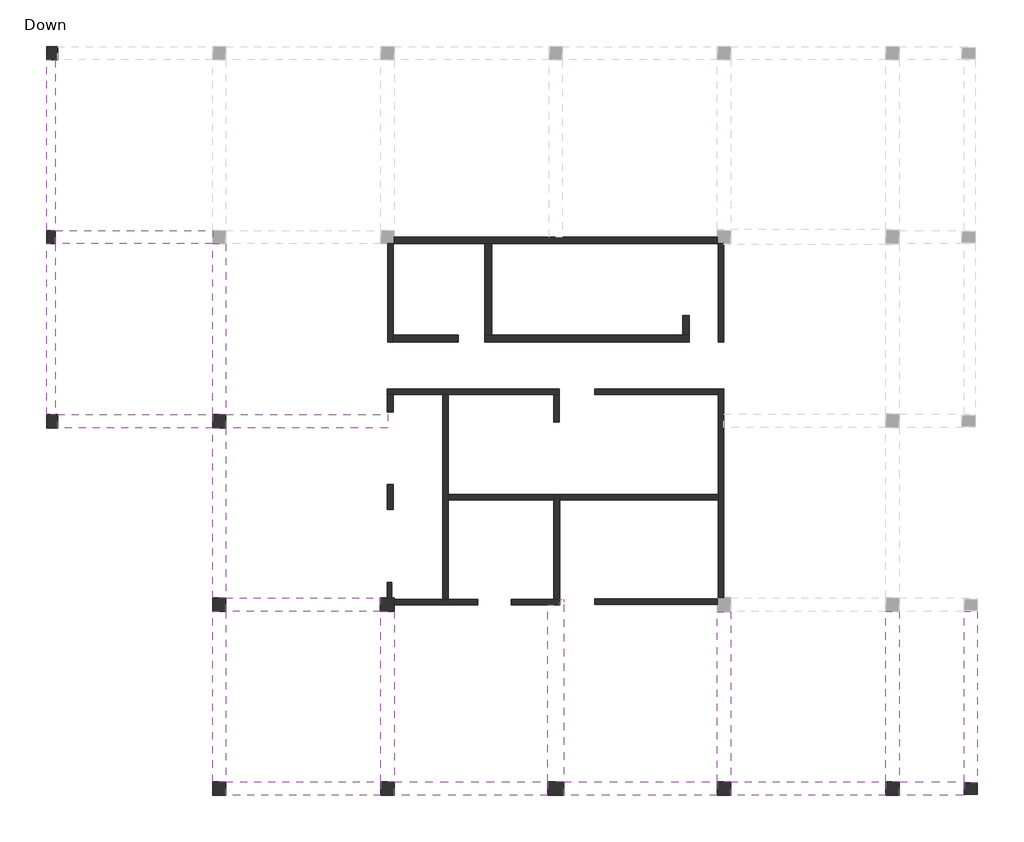
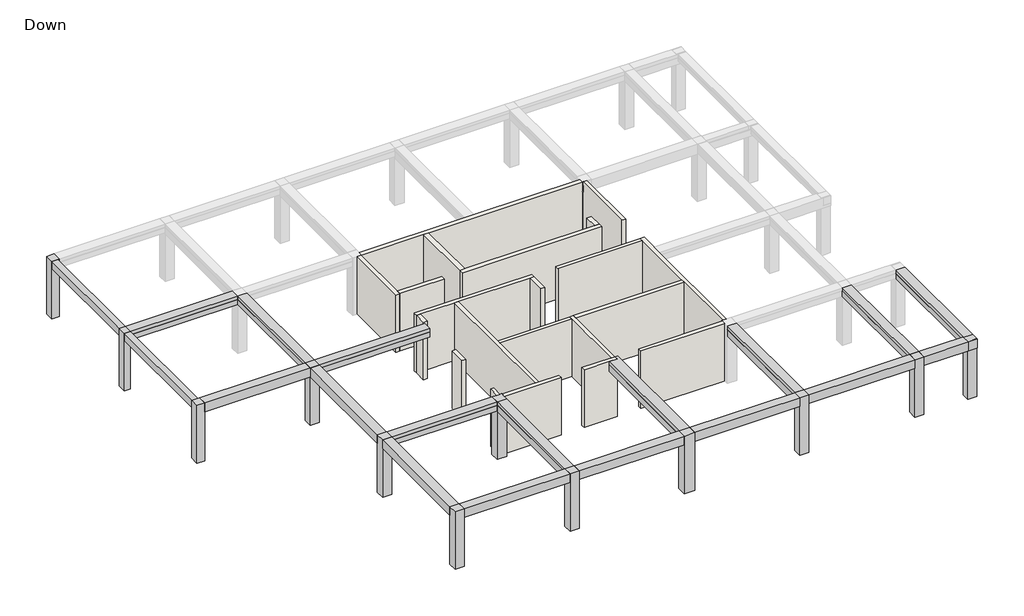
# One storey, part 1 of 2: 21 walls, 19 beams, 12 columns.
"""IFC4 building model written with IfcOpenShell, lengths in millimetres."""

from ifc_helpers import new_model, si_unit, frame, origin, origin_with_axes, place, context, project, spatial, polyline, outline, extrude, faceted_brep, element, save

model = new_model("IFC4")

# Units and contexts
model_context = context("Model", 3, world=origin())
ifc_project = project(units=[si_unit("LENGTHUNIT", "METRE", prefix="MILLI")], contexts=[model_context])

# Site, building, storey
site = spatial("IfcSite", under=ifc_project)
building = spatial("IfcBuilding", under=site)
storey = spatial("IfcBuildingStorey", under=building, Name="Down", Elevation=0.0)

# Beams
placement = place(None, origin())
element("IfcBeam", 1, ObjectType="Concrete Rectengular Beam : 40/50", at=placement, inside=storey, context=model_context, shape_type="SweptSolid", body=[
    extrude(outline(polyline([(4000.0, -21394.7160223), (3500.0, -21394.7160223), (3500.0, -20994.7160223), (3770.0, -20994.7160223), (3770.0, -20999.7160223), (4000.0, -20999.7160223), (4000.0, -21394.7160223)])), frame((0.0, 17936.6191558, 0.0), z_axis=(0.0, 1.0, 0.0), x_axis=(0.0, 0.0, 1.0)), (0.0, 0.0, 1.0), 7656.3440805),
])
element("IfcBeam", 2, ObjectType="Concrete Rectengular Beam : 40/50", at=placement, inside=storey, context=model_context, shape_type="SweptSolid", body=[
    extrude(outline(polyline([(4000.0, -21394.7160223), (3500.0, -21394.7160223), (3500.0, -20994.7160223), (3770.0, -20994.7160223), (3770.0, -20999.7160223), (4000.0, -20999.7160223), (4000.0, -21394.7160223)])), frame((0.0, 9666.6131842, 0.0), z_axis=(0.0, 1.0, 0.0), x_axis=(0.0, 0.0, 1.0)), (0.0, 0.0, 1.0), 7670.0059716),
])
element("IfcBeam", 3, ObjectType="Concrete Rectengular Beam : 60/60", at=placement, inside=storey, context=model_context, shape_type="SweptSolid", body=[
    extrude(outline(polyline([(3400.0, 16261.8802114), (3400.0, 16861.8802114), (3770.0, 16861.8802114), (3770.0, 16856.8802114), (4000.0, 16856.8802114), (4000.0, 16266.8802114), (3770.0, 16266.8802114), (3770.0, 16261.8802114), (3400.0, 16261.8802114)])), frame((0.0, -6825.0062825, 0.0), z_axis=(0.0, 1.0, 0.0), x_axis=(0.0, 0.0, 1.0)), (0.0, 0.0, 1.0), 7657.5072677),
])
element("IfcBeam", 4, ObjectType="Concrete Rectengular Beam : 60/60", at=placement, inside=storey, context=model_context, shape_type="SweptSolid", body=[
    extrude(outline(polyline([(-6825.0062825, 3400.0), (-7425.0062825, 3400.0), (-7425.0062825, 4000.0), (-6830.0062825, 4000.0), (-6830.0062825, 3770.0), (-6825.0062825, 3770.0), (-6825.0062825, 3400.0)])), frame((9303.3595467, 0.0, 0.0), z_axis=(1.0, 0.0, 0.0), x_axis=(0.0, 1.0, 0.0)), (0.0, 0.0, 1.0), 6958.5206647),
])
element("IfcBeam", 5, ObjectType="Concrete Rectengular Beam : 60/60", at=placement, inside=storey, context=model_context, shape_type="SweptSolid", body=[
    extrude(outline(polyline([(-6825.0062825, 3400.0), (-7425.0062825, 3400.0), (-7425.0062825, 4000.0), (-6830.0062825, 4000.0), (-6830.0062825, 3770.0), (-6825.0062825, 3770.0), (-6825.0062825, 3400.0)])), frame((1807.0810158, 0.0, 0.0), z_axis=(1.0, 0.0, 0.0), x_axis=(0.0, 1.0, 0.0)), (0.0, 0.0, 1.0), 6896.2785308),
])
element("IfcBeam", 6, ObjectType="Concrete Rectengular Beam : 60/60", at=placement, inside=storey, context=model_context, shape_type="SweptSolid", body=[
    extrude(outline(polyline([(-6825.0062825, 3400.0), (-7425.0062825, 3400.0), (-7425.0062825, 4000.0), (-6830.0062825, 4000.0), (-6830.0062825, 3770.0), (-6825.0062825, 3770.0), (-6825.0062825, 3400.0)])), frame((-5790.1585821, 0.0, 0.0), z_axis=(1.0, 0.0, 0.0), x_axis=(0.0, 1.0, 0.0)), (0.0, 0.0, 1.0), 6897.2395979),
])
element("IfcBeam", 7, ObjectType="Concrete Rectengular Beam : 60/60", at=placement, inside=storey, context=model_context, shape_type="SweptSolid", body=[
    extrude(outline(polyline([(-6825.0062825, 3400.0), (-7425.0062825, 3400.0), (-7425.0062825, 4000.0), (-6830.0062825, 4000.0), (-6830.0062825, 3770.0), (-6825.0062825, 3770.0), (-6825.0062825, 3400.0)])), frame((-13343.8144749, 0.0, 0.0), z_axis=(1.0, 0.0, 0.0), x_axis=(0.0, 1.0, 0.0)), (0.0, 0.0, 1.0), 6953.6558928),
])
element("IfcBeam", 8, ObjectType="Concrete Rectengular Beam : 60/60", at=placement, inside=storey, context=model_context, shape_type="SweptSolid", body=[
    extrude(outline(polyline([(4000.0, -13943.8144749), (3400.0, -13943.8144749), (3400.0, -13343.8144749), (3770.0, -13343.8144749), (3770.0, -13348.8144749), (4000.0, -13348.8144749), (4000.0, -13943.8144749)])), frame((0.0, -6825.0062825, 0.0), z_axis=(0.0, 1.0, 0.0), x_axis=(0.0, 0.0, 1.0)), (0.0, 0.0, 1.0), 7657.5072677),
])
element("IfcBeam", 9, ObjectType="Concrete Rectengular Beam : 60/60", at=placement, inside=storey, context=model_context, shape_type="SweptSolid", body=[
    extrude(outline(polyline([(3400.0, -13943.8144749), (3400.0, -13343.8144749), (3770.0, -13343.8144749), (3770.0, -13348.8144749), (4000.0, -13348.8144749), (4000.0, -13943.8144749), (3400.0, -13943.8144749)])), frame((0.0, 1432.5009852, 0.0), z_axis=(0.0, 1.0, 0.0), x_axis=(0.0, 0.0, 1.0)), (0.0, 0.0, 1.0), 7634.112199),
])
element("IfcBeam", 10, ObjectType="Concrete Rectengular Beam : 60/60", at=placement, inside=storey, context=model_context, shape_type="SweptSolid", body=[
    extrude(outline(polyline([(3400.0, -13943.8144749), (3400.0, -13343.8144749), (3770.0, -13343.8144749), (3770.0, -13348.8144749), (4000.0, -13348.8144749), (4000.0, -13938.8144749), (3770.0, -13938.8144749), (3770.0, -13943.8144749), (3400.0, -13943.8144749)])), frame((0.0, 9666.6131842, 0.0), z_axis=(0.0, 1.0, 0.0), x_axis=(0.0, 0.0, 1.0)), (0.0, 0.0, 1.0), 7670.0059716),
])
element("IfcBeam", 11, ObjectType="Concrete Rectengular Beam : 60/60", at=placement, inside=storey, context=model_context, shape_type="SweptSolid", body=[
    extrude(outline(polyline([(9666.6131842, 3400.0), (9066.6131842, 3400.0), (9066.6131842, 4000.0), (9661.6131842, 4000.0), (9661.6131842, 3770.0), (9666.6131842, 3770.0), (9666.6131842, 3400.0)])), frame((-20894.7160223, 0.0, 0.0), z_axis=(1.0, 0.0, 0.0), x_axis=(0.0, 1.0, 0.0)), (0.0, 0.0, 1.0), 6950.9015474),
])
element("IfcBeam", 12, ObjectType="Concrete Rectengular Beam : 60/60", at=placement, inside=storey, context=model_context, shape_type="SweptSolid", body=[
    extrude(outline(polyline([(17936.6191558, 3400.0), (17336.6191558, 3400.0), (17336.6191558, 3770.0), (17341.6191558, 3770.0), (17341.6191558, 4000.0), (17931.6191558, 4000.0), (17931.6191558, 3770.0), (17936.6191558, 3770.0), (17936.6191558, 3400.0)])), frame((-20994.7160223, 0.0, 0.0), z_axis=(1.0, 0.0, 0.0), x_axis=(0.0, 1.0, 0.0)), (0.0, 0.0, 1.0), 7050.9015474),
])
element("IfcBeam", 13, ObjectType="Concrete Rectengular Beam : 60/60", at=placement, inside=storey, context=model_context, shape_type="SweptSolid", body=[
    extrude(outline(polyline([(9666.6131842, 3400.0), (9066.6131842, 3400.0), (9066.6131842, 3770.0), (9071.6131842, 3770.0), (9071.6131842, 4000.0), (9661.6131842, 4000.0), (9661.6131842, 3770.0), (9666.6131842, 3770.0), (9666.6131842, 3400.0)])), frame((-13343.8144749, 0.0, 0.0), z_axis=(1.0, 0.0, 0.0), x_axis=(0.0, 1.0, 0.0)), (0.0, 0.0, 1.0), 7253.6558928),
])
element("IfcBeam", 14, ObjectType="Concrete Rectengular Beam : 60/60", at=placement, inside=storey, context=model_context, shape_type="SweptSolid", body=[
    extrude(outline(polyline([(1432.5009852, 3400.0), (832.5009852, 3400.0), (832.5009852, 3770.0), (837.5009852, 3770.0), (837.5009852, 4000.0), (1430.5203801, 4000.0), (1430.5203801, 3770.0), (1432.5009852, 3770.0), (1432.5009852, 3400.0)])), frame((-13343.8144749, 0.0, 0.0), z_axis=(1.0, 0.0, 0.0), x_axis=(0.0, 1.0, 0.0)), (0.0, 0.0, 1.0), 6919.0299628),
])
element("IfcBeam", 15, ObjectType="Concrete Rectengular Beam : 60/60", at=placement, inside=storey, context=model_context, shape_type="Brep", body=[
    faceted_brep([(19778.1411959, -7425.0062825, 4000.0), (20378.1412457, -7425.0062825, 4000.0), (20378.1616289, -7375.0062825, 4000.0), (19778.1615791, -7375.0062825, 4000.0), (19778.1411959, -7425.0062825, 3400.0), (19778.1615791, -7375.0062825, 3400.0), (20378.1412457, -7425.0062825, 3400.0), (20378.1616289, -7375.0062825, 3400.0)], [[[0, 1, 2, 3]], [[4, 0, 3, 5]], [[6, 4, 5, 7]], [[1, 6, 7, 2]], [[1, 0, 4, 6]], [[3, 2, 7, 5]]]),
    faceted_brep([(20381.5075349, 832.5009852, 3400.0), (19781.507485, 832.5009852, 3400.0), (19781.507485, 832.5009852, 3770.0), (19786.5074854, 832.5009852, 3770.0), (19786.5074854, 832.5009852, 4000.0), (20381.5075349, 832.5009852, 4000.0), (19778.3857943, -6825.0062825, 3770.0), (19778.383756, -6830.0062825, 3770.0), (19783.3837564, -6830.0062825, 3770.0), (19783.3837564, -6830.0062825, 4000.0), (19778.383756, -6830.0062825, 4000.0), (20378.365461, -6875.0062825, 4000.0), (19778.3654111, -6875.0062825, 4000.0), (19778.3654111, -6875.0062825, 3400.0), (20378.365461, -6875.0062825, 3400.0), (19778.3857943, -6825.0062825, 3400.0)], [[[0, 1, 2, 3, 4, 5]], [[2, 6, 7, 8, 3]], [[8, 9, 4, 3]], [[9, 8, 7, 10]], [[11, 12, 13, 14]], [[4, 9, 10, 12, 11, 5]], [[10, 7, 6, 2, 1, 15, 13, 12]], [[1, 0, 14, 13, 15]], [[0, 5, 11, 14]]]),
])
element("IfcBeam", 16, ObjectType="Concrete Rectengular Beam : 60/60", at=placement, inside=storey, context=model_context, shape_type="Brep", body=[
    faceted_brep([(16861.8802114, -7425.0062825, 4000.0), (19778.1411959, -7425.0062825, 4000.0), (19778.3654111, -6875.0062825, 4000.0), (19778.383756, -6830.0062825, 4000.0), (16861.8802114, -6830.0062825, 4000.0), (19778.3857943, -6825.0062825, 3400.0), (16861.8802114, -6825.0062825, 3400.0), (16861.8802114, -6825.0062825, 3770.0), (19778.3857943, -6825.0062825, 3770.0), (19778.3654111, -6875.0062825, 3400.0), (19778.1411959, -7425.0062825, 3400.0), (16861.8802114, -7425.0062825, 3400.0), (16861.8802114, -6830.0062825, 3770.0), (19778.383756, -6830.0062825, 3770.0)], [[[0, 1, 2, 3, 4]], [[5, 6, 7, 8]], [[5, 9, 10, 11, 6]], [[0, 11, 10, 1]], [[11, 0, 4, 12, 7, 6]], [[10, 9, 5, 8, 13, 3, 2, 1]], [[12, 13, 8, 7]], [[13, 12, 4, 3]]]),
])
element("IfcBeam", 17, ObjectType="Concrete Rectengular Beam : 60/70", at=placement, inside=storey, context=model_context, shape_type="SweptSolid", body=[
    extrude(outline(polyline([(3300.0, -6390.1585821), (3300.0, -5790.1585821), (3770.0, -5790.1585821), (3770.0, -5795.1585821), (4000.0, -5795.1585821), (4000.0, -6385.1585821), (3770.0, -6385.1585821), (3770.0, -6390.1585821), (3300.0, -6390.1585821)])), frame((0.0, -6825.0062825, 0.0), z_axis=(0.0, 1.0, 0.0), x_axis=(0.0, 0.0, 1.0)), (0.0, 0.0, 1.0), 7657.5072677),
])
element("IfcBeam", 18, ObjectType="Concrete Rectengular Beam : 60/70", at=placement, inside=storey, context=model_context, shape_type="SweptSolid", body=[
    extrude(outline(polyline([(3300.0, 8703.3595467), (3300.0, 9303.3595467), (3770.0, 9303.3595467), (3770.0, 9298.3595467), (4000.0, 9298.3595467), (4000.0, 8708.3595467), (3770.0, 8708.3595467), (3770.0, 8703.3595467), (3300.0, 8703.3595467)])), frame((0.0, -6825.0062825, 0.0), z_axis=(0.0, 1.0, 0.0), x_axis=(0.0, 0.0, 1.0)), (0.0, 0.0, 1.0), 7637.5072677),
])
element("IfcBeam", 19, ObjectType="Concrete Rectengular Beam : 70/70", at=placement, inside=storey, context=model_context, shape_type="Brep", body=[
    faceted_brep([(1807.0810158, 1138.5687304, 4000.0), (1807.0810158, 1377.9140303, 4000.0), (1628.3544453, 1377.9140303, 4000.0), (1628.3544453, 1127.9140303, 4000.0), (1112.0810158, 1127.9140303, 4000.0), (1112.0810158, -6825.0062825, 4000.0), (1802.0810158, -6825.0062825, 4000.0), (1802.0810158, 1138.5687304, 4000.0), (1807.0810158, 1377.9140303, 3300.0), (1807.0810158, 1138.5687304, 3770.0), (1807.0810158, -6825.0062825, 3770.0), (1807.0810158, -6825.0062825, 3300.0), (1107.0810158, -6825.0062825, 3300.0), (1107.0810158, 1127.9140303, 3300.0), (1628.3544453, 1127.9140303, 3300.0), (1628.3544453, 1377.9140303, 3300.0), (1107.0810158, -6825.0062825, 3770.0), (1107.0810158, 1127.9140303, 3770.0), (1802.0810158, -6825.0062825, 3770.0), (1112.0810158, -6825.0062825, 3770.0), (1112.0810158, 1127.9140303, 3770.0), (1802.0810158, 1138.5687304, 3770.0)], [[[0, 1, 2, 3, 4, 5, 6, 7]], [[8, 1, 0, 9, 10, 11]], [[11, 12, 13, 14, 15, 8]], [[12, 16, 17, 13]], [[12, 11, 10, 18, 6, 5, 19, 16]], [[1, 8, 15, 2]], [[16, 19, 20, 17]], [[19, 5, 4, 20]], [[21, 18, 10, 9]], [[7, 21, 9, 0]], [[21, 7, 6, 18]], [[3, 14, 13, 17, 20, 4]], [[14, 3, 2, 15]]]),
])

# Columns
element("IfcColumn", 20, ObjectType="Concrete Rectengular Column : 60/40", at=placement, inside=storey, context=model_context, shape_type="Brep", body=[
    faceted_brep([(-21394.7160223, 17936.6191558, 0.0), (-20994.7160223, 17936.6191558, 0.0), (-20994.7160223, 17336.6191558, 0.0), (-21394.7160223, 17336.6191558, 0.0), (-21394.7160223, 17936.6191558, 4000.0), (-20999.7160223, 17936.6191558, 4000.0), (-20994.7160223, 17936.6191558, 4000.0), (-20994.7160223, 17936.6191558, 3770.0), (-20994.7160223, 17931.6191558, 4000.0), (-20994.7160223, 17341.6191558, 4000.0), (-20994.7160223, 17336.6191558, 4000.0), (-20994.7160223, 17336.6191558, 3770.0), (-20999.7160223, 17336.6191558, 4000.0), (-21394.7160223, 17336.6191558, 4000.0)], [[[0, 1, 2, 3]], [[4, 5, 6, 7, 1, 0]], [[6, 8, 9, 10, 11, 2, 1, 7]], [[10, 12, 13, 3, 2, 11]], [[13, 4, 0, 3]], [[4, 13, 12, 10, 9, 8, 6, 5]]]),
])
element("IfcColumn", 21, ObjectType="Concrete Rectengular Column : 60/50", at=placement, inside=storey, context=model_context, shape_type="Brep", body=[
    faceted_brep([(-21394.7160223, 9666.6131842, 0.0), (-20894.7160223, 9666.6131842, 0.0), (-20894.7160223, 9066.6131842, 0.0), (-21394.7160223, 9066.6131842, 0.0), (-21394.7160223, 9666.6131842, 4000.0), (-20999.7160223, 9666.6131842, 4000.0), (-20894.7160223, 9666.6131842, 4000.0), (-20894.7160223, 9666.6131842, 3770.0), (-20894.7160223, 9661.6131842, 4000.0), (-20894.7160223, 9066.6131842, 4000.0), (-21394.7160223, 9066.6131842, 4000.0)], [[[0, 1, 2, 3]], [[4, 5, 6, 7, 1, 0]], [[6, 8, 9, 2, 1, 7]], [[9, 10, 3, 2]], [[10, 4, 0, 3]], [[4, 10, 9, 8, 6, 5]]]),
])
element("IfcColumn", 22, ObjectType="Concrete Rectengular Column : 60/50", at=placement, inside=storey, context=model_context, shape_type="Brep", body=[
    faceted_brep([(-21394.7160223, 26192.9632364, 0.0), (-20894.7160223, 26192.9632364, 0.0), (-20894.7160223, 25592.9632364, 0.0), (-21394.7160223, 25592.9632364, 0.0), (-21394.7160223, 26192.9632364, 4000.0), (-20894.7160223, 26192.9632364, 4000.0), (-20894.7160223, 25597.9632364, 4000.0), (-20894.7160223, 25592.9632364, 4000.0), (-20894.7160223, 25592.9632364, 3770.0), (-20999.7160223, 25592.9632364, 4000.0), (-21394.7160223, 25592.9632364, 4000.0)], [[[0, 1, 2, 3]], [[4, 5, 1, 0]], [[5, 6, 7, 8, 2, 1]], [[7, 9, 10, 3, 2, 8]], [[10, 4, 0, 3]], [[4, 10, 9, 7, 6, 5]]]),
])
element("IfcColumn", 23, ObjectType="Concrete Rectengular Column : 60/50", at=placement, inside=storey, context=model_context, shape_type="SweptSolid", body=[
    extrude(outline(polyline([(20378.26352, -6875.0062825), (20378.26352, -7375.0062825), (19778.26352, -7375.0062825), (19778.26352, -6875.0062825), (20378.26352, -6875.0062825)])), origin_with_axes(), (0.0, 0.0, 1.0), 4000.0),
])
element("IfcColumn", 24, ObjectType="Concrete Rectengular Column : 60/60", at=placement, inside=storey, context=model_context, shape_type="Brep", body=[
    faceted_brep([(-13343.8144749, 9666.6131842, 0.0), (-13343.8144749, 9066.6131842, 0.0), (-13943.8144749, 9066.6131842, 0.0), (-13943.8144749, 9666.6131842, 0.0), (-13343.8144749, 9666.6131842, 4000.0), (-13343.8144749, 9661.6131842, 4000.0), (-13343.8144749, 9071.6131842, 4000.0), (-13343.8144749, 9066.6131842, 4000.0), (-13343.8144749, 9066.6131842, 3770.0), (-13343.8144749, 9666.6131842, 3770.0), (-13348.8144749, 9066.6131842, 4000.0), (-13943.8144749, 9066.6131842, 4000.0), (-13943.8144749, 9661.6131842, 4000.0), (-13943.8144749, 9666.6131842, 4000.0), (-13943.8144749, 9666.6131842, 3770.0), (-13938.8144749, 9666.6131842, 4000.0), (-13348.8144749, 9666.6131842, 4000.0)], [[[0, 1, 2, 3]], [[4, 5, 6, 7, 8, 1, 0, 9]], [[7, 10, 11, 2, 1, 8]], [[11, 12, 13, 14, 3, 2]], [[13, 15, 16, 4, 9, 0, 3, 14]], [[4, 16, 15, 13, 12, 11, 10, 7, 6, 5]]]),
])
element("IfcColumn", 25, ObjectType="Concrete Rectengular Column : 60/60", at=placement, inside=storey, context=model_context, shape_type="Brep", body=[
    faceted_brep([(-13343.8144749, 1432.5009852, 0.0), (-13343.8144749, 832.5009852, 0.0), (-13943.8144749, 832.5009852, 0.0), (-13943.8144749, 1432.5009852, 0.0), (-13343.8144749, 1432.5009852, 4000.0), (-13343.8144749, 1430.5203801, 4000.0), (-13343.8144749, 837.5009852, 4000.0), (-13343.8144749, 832.5009852, 4000.0), (-13343.8144749, 832.5009852, 3770.0), (-13343.8144749, 1432.5009852, 3770.0), (-13348.8144749, 832.5009852, 4000.0), (-13943.8144749, 832.5009852, 4000.0), (-13943.8144749, 1432.5009852, 4000.0), (-13348.8144749, 1432.5009852, 4000.0)], [[[0, 1, 2, 3]], [[4, 5, 6, 7, 8, 1, 0, 9]], [[7, 10, 11, 2, 1, 8]], [[11, 12, 3, 2]], [[12, 13, 4, 9, 0, 3]], [[4, 13, 12, 11, 10, 7, 6, 5]]]),
])
element("IfcColumn", 26, ObjectType="Concrete Rectengular Column : 60/60", at=placement, inside=storey, context=model_context, shape_type="Brep", body=[
    faceted_brep([(-13343.8144749, -6825.0062825, 0.0), (-13343.8144749, -7425.0062825, 0.0), (-13943.8144749, -7425.0062825, 0.0), (-13943.8144749, -6825.0062825, 0.0), (-13343.8144749, -6825.0062825, 4000.0), (-13343.8144749, -6830.0062825, 4000.0), (-13343.8144749, -7425.0062825, 4000.0), (-13343.8144749, -6825.0062825, 3770.0), (-13943.8144749, -7425.0062825, 4000.0), (-13943.8144749, -6825.0062825, 4000.0), (-13348.8144749, -6825.0062825, 4000.0)], [[[0, 1, 2, 3]], [[4, 5, 6, 1, 0, 7]], [[6, 8, 2, 1]], [[8, 9, 3, 2]], [[9, 10, 4, 7, 0, 3]], [[4, 10, 9, 8, 6, 5]]]),
])
element("IfcColumn", 27, ObjectType="Concrete Rectengular Column : 60/60", at=placement, inside=storey, context=model_context, shape_type="Brep", body=[
    faceted_brep([(-5790.1585821, -6825.0062825, 0.0), (-5790.1585821, -7425.0062825, 0.0), (-6390.1585821, -7425.0062825, 0.0), (-6390.1585821, -6825.0062825, 0.0), (-5790.1585821, -6825.0062825, 4000.0), (-5790.1585821, -6830.0062825, 4000.0), (-5790.1585821, -7425.0062825, 4000.0), (-5790.1585821, -6825.0062825, 3770.0), (-6390.1585821, -7425.0062825, 4000.0), (-6390.1585821, -6830.0062825, 4000.0), (-6390.1585821, -6825.0062825, 4000.0), (-6390.1585821, -6825.0062825, 3770.0), (-6385.1585821, -6825.0062825, 4000.0), (-5795.1585821, -6825.0062825, 4000.0)], [[[0, 1, 2, 3]], [[4, 5, 6, 1, 0, 7]], [[6, 8, 2, 1]], [[8, 9, 10, 11, 3, 2]], [[10, 12, 13, 4, 7, 0, 3, 11]], [[4, 13, 12, 10, 9, 8, 6, 5]]]),
])
element("IfcColumn", 28, ObjectType="Concrete Rectengular Column : 60/60", at=placement, inside=storey, context=model_context, shape_type="Brep", body=[
    faceted_brep([(8703.3595467, -6825.0062825, 0.0), (9303.3595467, -6825.0062825, 0.0), (9303.3595467, -7425.0062825, 0.0), (8703.3595467, -7425.0062825, 0.0), (8703.3595467, -6825.0062825, 4000.0), (8708.3595467, -6825.0062825, 4000.0), (9298.3595467, -6825.0062825, 4000.0), (9303.3595467, -6825.0062825, 4000.0), (9303.3595467, -6825.0062825, 3770.0), (8703.3595467, -6825.0062825, 3770.0), (9303.3595467, -6830.0062825, 4000.0), (9303.3595467, -7425.0062825, 4000.0), (8703.3595467, -7425.0062825, 4000.0), (8703.3595467, -6830.0062825, 4000.0)], [[[0, 1, 2, 3]], [[4, 5, 6, 7, 8, 1, 0, 9]], [[7, 10, 11, 2, 1, 8]], [[11, 12, 3, 2]], [[12, 13, 4, 9, 0, 3]], [[4, 13, 12, 11, 10, 7, 6, 5]]]),
])
element("IfcColumn", 29, ObjectType="Concrete Rectengular Column : 60/60", at=placement, inside=storey, context=model_context, shape_type="Brep", body=[
    faceted_brep([(16261.8802114, -6825.0062825, 0.0), (16861.8802114, -6825.0062825, 0.0), (16861.8802114, -7425.0062825, 0.0), (16261.8802114, -7425.0062825, 0.0), (16261.8802114, -6825.0062825, 4000.0), (16266.8802114, -6825.0062825, 4000.0), (16861.8802114, -6825.0062825, 4000.0), (16861.8802114, -6825.0062825, 3770.0), (16261.8802114, -6825.0062825, 3770.0), (16861.8802114, -7425.0062825, 4000.0), (16261.8802114, -7425.0062825, 4000.0), (16261.8802114, -6830.0062825, 4000.0)], [[[0, 1, 2, 3]], [[4, 5, 6, 7, 1, 0, 8]], [[6, 9, 2, 1, 7]], [[9, 10, 3, 2]], [[10, 11, 4, 8, 0, 3]], [[4, 11, 10, 9, 6, 5]]]),
])
element("IfcColumn", 30, ObjectType="Concrete Rectengular Column : 60/70", at=placement, inside=storey, context=model_context, shape_type="Brep", body=[
    faceted_brep([(1107.0810158, -6825.0062825, 0.0), (1807.0810158, -6825.0062825, 0.0), (1807.0810158, -7425.0062825, 0.0), (1107.0810158, -7425.0062825, 0.0), (1107.0810158, -6825.0062825, 4000.0), (1112.0810158, -6825.0062825, 4000.0), (1802.0810158, -6825.0062825, 4000.0), (1807.0810158, -6825.0062825, 4000.0), (1807.0810158, -6825.0062825, 3770.0), (1107.0810158, -6825.0062825, 3770.0), (1807.0810158, -6830.0062825, 4000.0), (1807.0810158, -7425.0062825, 4000.0), (1107.0810158, -7425.0062825, 4000.0), (1107.0810158, -6830.0062825, 4000.0)], [[[0, 1, 2, 3]], [[4, 5, 6, 7, 8, 1, 0, 9]], [[7, 10, 11, 2, 1, 8]], [[11, 12, 3, 2]], [[12, 13, 4, 9, 0, 3]], [[4, 13, 12, 11, 10, 7, 6, 5]]]),
])
element("IfcColumn", 31, ObjectType="Concrete Rectengular Column : 64/60", at=placement, inside=storey, context=model_context, shape_type="Brep", body=[
    faceted_brep([(-5784.7845121, 1432.5009852, 0.0), (-5784.7845121, 1377.9140303, 0.0), (-5784.7845121, 1127.9140303, 0.0), (-5784.7845121, 832.5009852, 0.0), (-6424.7845121, 832.5009852, 0.0), (-6424.7845121, 1432.5009852, 0.0), (-6098.8711202, 1432.5009852, 0.0), (-5898.8711202, 1432.5009852, 0.0), (-5784.7845121, 1432.5009852, 4000.0), (-5784.7845121, 1377.9140303, 4000.0), (-5784.7845121, 1127.9140303, 4000.0), (-5784.7845121, 832.5009852, 4000.0), (-5784.7845121, 832.5009852, 3770.0), (-5795.1585821, 832.5009852, 4000.0), (-6385.1585821, 832.5009852, 4000.0), (-6424.7845121, 832.5009852, 4000.0), (-6424.7845121, 832.5009852, 3770.0), (-6424.7845121, 837.5009852, 4000.0), (-6424.7845121, 1430.5203801, 4000.0), (-6424.7845121, 1432.5009852, 4000.0), (-6424.7845121, 1432.5009852, 3770.0), (-6098.8711202, 1432.5009852, 4000.0), (-5898.8711202, 1432.5009852, 4000.0)], [[[0, 1, 2, 3, 4, 5, 6, 7]], [[8, 9, 10, 11, 12, 3, 2, 1, 0]], [[11, 13, 14, 15, 16, 4, 3, 12]], [[15, 17, 18, 19, 20, 5, 4, 16]], [[19, 21, 22, 8, 0, 7, 6, 5, 20]], [[8, 22, 21, 19, 18, 17, 15, 14, 13, 11, 10, 9]]]),
])

# Walls
element("IfcWall", 32, ObjectType="20", at=placement, inside=storey, context=model_context, shape_type="Brep", body=[
    faceted_brep([(-5898.8711202, 1432.5009852, 0.0), (-5898.8711202, 2140.5203801, 0.0), (-5898.8711202, 2140.5203801, 4000.0), (-5898.8711202, 1432.5009852, 4000.0), (-6098.8711202, 1432.5009852, 0.0), (-6098.8711202, 1432.5009852, 3770.0), (-6098.8711202, 1432.5009852, 4000.0), (-6098.8711202, 2140.5203801, 4000.0), (-6098.8711202, 2140.5203801, 3770.0), (-6098.8711202, 2140.5203801, 0.0)], [[[0, 1, 2, 3]], [[4, 5, 6, 7, 8, 9]], [[1, 0, 4, 9]], [[2, 1, 9, 8, 7]], [[3, 2, 7, 6]], [[0, 3, 6, 5, 4]]]),
])
element("IfcWall", 33, ObjectType="25", at=placement, inside=storey, context=model_context, shape_type="Brep", body=[
    faceted_brep([(8756.9599651, 17336.6191558, 0.0), (8756.9599651, 12927.509382, 0.0), (8756.9599651, 12927.509382, 3770.0), (8756.9599651, 12927.509382, 4000.0), (8756.9599651, 17336.6191558, 4000.0), (8756.9599651, 17336.6191558, 3770.0), (8756.9599651, 17336.6191558, 3350.0), (8756.9599651, 17336.6191558, 3300.0), (9006.9599651, 17336.6191558, 0.0), (9006.9599651, 17336.6191558, 3300.0), (9006.9599651, 17336.6191558, 3350.0), (9006.9599651, 17336.6191558, 4000.0), (9006.9599651, 17293.0356779, 4000.0), (9006.9599651, 12927.509382, 4000.0), (9006.9599651, 12927.509382, 3770.0), (9006.9599651, 12927.509382, 0.0), (9003.3595467, 12927.509382, 4000.0)], [[[0, 1, 2, 3, 4, 5, 6, 7]], [[8, 9, 10, 11, 12, 13, 14, 15]], [[1, 0, 8, 15]], [[3, 2, 1, 15, 14, 13, 16]], [[4, 3, 16, 13, 12, 11]], [[0, 7, 6, 5, 4, 11, 10, 9, 8]]]),
])
element("IfcWall", 34, ObjectType="25", at=placement, inside=storey, context=model_context, shape_type="Brep", body=[
    faceted_brep([(-6090.1585821, 17336.6191558, 0.0), (-6090.1585821, 12927.509382, 0.0), (-6090.1585821, 12927.509382, 3770.0), (-6090.1585821, 12927.509382, 4000.0), (-6090.1585821, 17336.6191558, 4000.0), (-6090.1585821, 17336.6191558, 3770.0), (-5840.1585821, 17336.6191558, 0.0), (-5840.1585821, 17336.6191558, 3770.0), (-5840.1585821, 17336.6191558, 4000.0), (-5840.1585821, 13227.509382, 4000.0), (-5840.1585821, 12927.509382, 4000.0), (-5840.1585821, 12927.509382, 0.0), (-5840.1585821, 13227.509382, 0.0), (-6084.2021017, 12927.509382, 4000.0)], [[[0, 1, 2, 3, 4, 5]], [[6, 7, 8, 9, 10, 11, 12]], [[1, 0, 6, 12, 11]], [[4, 3, 13, 10, 9, 8]], [[0, 5, 4, 8, 7, 6]], [[3, 2, 1, 11, 10, 13]]]),
])
element("IfcWall", 35, ObjectType="25", at=placement, inside=storey, context=model_context, shape_type="Brep", body=[
    faceted_brep([(-5784.7845121, 1127.9140303, 0.0), (-2044.60675, 1127.9140303, 0.0), (-2044.60675, 1127.9140303, 3770.0), (-2044.60675, 1127.9140303, 4000.0), (-5784.7845121, 1127.9140303, 4000.0), (-5784.7845121, 1127.9140303, 3770.0), (-5784.7845121, 1377.9140303, 0.0), (-5784.7845121, 1377.9140303, 4000.0), (-3606.6009397, 1377.9140303, 4000.0), (-3356.6009397, 1377.9140303, 4000.0), (-2044.60675, 1377.9140303, 4000.0), (-2044.60675, 1377.9140303, 3770.0), (-2044.60675, 1377.9140303, 0.0), (-3356.6009397, 1377.9140303, 0.0), (-3606.6009397, 1377.9140303, 0.0), (-2044.60675, 1132.9140303, 4000.0)], [[[0, 1, 2, 3, 4, 5]], [[6, 7, 8, 9, 10, 11, 12, 13, 14]], [[1, 0, 6, 14, 13, 12]], [[3, 2, 1, 12, 11, 10, 15]], [[4, 3, 15, 10, 9, 8, 7]], [[0, 5, 4, 7, 6]]]),
])
element("IfcWall", 36, ObjectType="25", at=placement, inside=storey, context=model_context, shape_type="Brep", body=[
    faceted_brep([(-534.9574452, 1127.9140303, 0.0), (1628.3544453, 1127.9140303, 0.0), (1628.3544453, 1127.9140303, 3300.0), (1628.3544453, 1127.9140303, 4000.0), (1112.0810158, 1127.9140303, 4000.0), (-534.9574452, 1127.9140303, 4000.0), (-534.9574452, 1127.9140303, 3770.0), (-534.9574452, 1377.9140303, 0.0), (-534.9574452, 1377.9140303, 3770.0), (-534.9574452, 1377.9140303, 4000.0), (1378.3544453, 1377.9140303, 4000.0), (1628.3544453, 1377.9140303, 4000.0), (1628.3544453, 1377.9140303, 3300.0), (1628.3544453, 1377.9140303, 0.0), (1378.3544453, 1377.9140303, 0.0), (-534.9574452, 1132.9140303, 4000.0)], [[[0, 1, 2, 3, 4, 5, 6]], [[7, 8, 9, 10, 11, 12, 13, 14]], [[1, 0, 7, 14, 13]], [[5, 4, 3, 11, 10, 9, 15]], [[0, 6, 5, 15, 9, 8, 7]], [[3, 2, 1, 13, 12, 11]]]),
])
element("IfcWall", 37, ObjectType="25", at=placement, inside=storey, context=model_context, shape_type="Brep", body=[
    faceted_brep([(1628.3544453, 1377.9140303, 0.0), (1628.3544453, 5836.2983934, 0.0), (1628.3544453, 6086.2983934, 0.0), (1628.3544453, 6086.2983934, 4000.0), (1628.3544453, 5836.2983934, 4000.0), (1628.3544453, 1377.9140303, 4000.0), (1378.3544453, 1377.9140303, 0.0), (1378.3544453, 1377.9140303, 3770.0), (1378.3544453, 1377.9140303, 4000.0), (1378.3544453, 5836.2983934, 4000.0), (1378.3544453, 6086.2983934, 4000.0), (1378.3544453, 6086.2983934, 0.0), (1378.3544453, 5836.2983934, 0.0)], [[[0, 1, 2, 3, 4, 5]], [[6, 7, 8, 9, 10, 11, 12]], [[2, 1, 0, 6, 12, 11]], [[5, 4, 3, 10, 9, 8]], [[0, 5, 8, 7, 6]], [[3, 2, 11, 10]]]),
])
element("IfcWall", 38, ObjectType="25", at=placement, inside=storey, context=model_context, shape_type="Brep", body=[
    faceted_brep([(1628.3544453, 5836.2983934, 0.0), (8756.9599651, 5836.2983934, 0.0), (8756.9599651, 5836.2983934, 4000.0), (1628.3544453, 5836.2983934, 4000.0), (1628.3544453, 6086.2983934, 0.0), (1628.3544453, 6086.2983934, 4000.0), (8756.9599651, 6086.2983934, 4000.0), (8756.9599651, 6086.2983934, 3770.0), (8756.9599651, 6086.2983934, 0.0)], [[[0, 1, 2, 3]], [[4, 5, 6, 7, 8]], [[1, 0, 4, 8]], [[3, 2, 6, 5]], [[0, 3, 5, 4]], [[2, 1, 8, 7, 6]]]),
])
element("IfcWall", 39, ObjectType="25", at=placement, inside=storey, context=model_context, shape_type="Brep", body=[
    faceted_brep([(9006.9599651, 1457.2873442, 0.0), (9006.9599651, 10823.3383922, 0.0), (9006.9599651, 10823.3383922, 3770.0), (9006.9599651, 10823.3383922, 4000.0), (9006.9599651, 9681.6131842, 4000.0), (9006.9599651, 9086.6131842, 4000.0), (9006.9599651, 1457.2873442, 4000.0), (9006.9599651, 1457.2873442, 3770.0), (8756.9599651, 1457.2873442, 0.0), (8756.9599651, 1457.2873442, 4000.0), (8756.9599651, 5836.2983934, 4000.0), (8756.9599651, 6086.2983934, 4000.0), (8756.9599651, 10573.3383922, 4000.0), (8756.9599651, 10823.3383922, 4000.0), (8756.9599651, 10823.3383922, 0.0), (8756.9599651, 10573.3383922, 0.0), (8756.9599651, 6086.2983934, 0.0), (8756.9599651, 5836.2983934, 0.0), (9003.3595467, 10823.3383922, 4000.0), (9001.9599651, 1457.2873442, 4000.0)], [[[0, 1, 2, 3, 4, 5, 6, 7]], [[8, 9, 10, 11, 12, 13, 14, 15, 16, 17]], [[1, 0, 8, 17, 16, 15, 14]], [[6, 5, 4, 3, 18, 13, 12, 11, 10, 9, 19]], [[0, 7, 6, 19, 9, 8]], [[3, 2, 1, 14, 13, 18]]]),
])
element("IfcWall", 40, ObjectType="25", at=placement, inside=storey, context=model_context, shape_type="Brep", body=[
    faceted_brep([(8756.9599651, 10823.3383922, 0.0), (3208.0390271, 10823.3383922, 0.0), (3208.0390271, 10823.3383922, 3770.0), (3208.0390271, 10823.3383922, 4000.0), (8756.9599651, 10823.3383922, 4000.0), (8756.9599651, 10573.3383922, 0.0), (8756.9599651, 10573.3383922, 3770.0), (8756.9599651, 10573.3383922, 4000.0), (3208.0390271, 10573.3383922, 4000.0), (3208.0390271, 10573.3383922, 3770.0), (3208.0390271, 10573.3383922, 0.0), (3208.0390271, 10593.3383922, 4000.0)], [[[0, 1, 2, 3, 4]], [[5, 6, 7, 8, 9, 10]], [[1, 0, 5, 10]], [[3, 2, 1, 10, 9, 8, 11]], [[4, 3, 11, 8, 7]], [[0, 4, 7, 6, 5]]]),
])
element("IfcWall", 41, ObjectType="25", at=placement, inside=storey, context=model_context, shape_type="Brep", body=[
    faceted_brep([(1622.1290873, 10823.3383922, 0.0), (-6094.2021017, 10823.3383922, 0.0), (-6094.2021017, 10823.3383922, 3770.0), (-6094.2021017, 10823.3383922, 4000.0), (-6084.2021017, 10823.3383922, 4000.0), (1622.1290873, 10823.3383922, 4000.0), (1622.1290873, 10823.3383922, 3770.0), (1622.1290873, 10573.3383922, 0.0), (1622.1290873, 10573.3383922, 4000.0), (1372.1290873, 10573.3383922, 4000.0), (-3356.6009397, 10573.3383922, 4000.0), (-3606.6009397, 10573.3383922, 4000.0), (-5844.2021017, 10573.3383922, 4000.0), (-6094.2021017, 10573.3383922, 4000.0), (-6094.2021017, 10573.3383922, 0.0), (-5844.2021017, 10573.3383922, 0.0), (-3606.6009397, 10573.3383922, 0.0), (-3356.6009397, 10573.3383922, 0.0), (1372.1290873, 10573.3383922, 0.0), (1622.1290873, 10593.3383922, 4000.0)], [[[0, 1, 2, 3, 4, 5, 6]], [[7, 8, 9, 10, 11, 12, 13, 14, 15, 16, 17, 18]], [[1, 0, 7, 18, 17, 16, 15, 14]], [[5, 4, 3, 13, 12, 11, 10, 9, 8, 19]], [[3, 2, 1, 14, 13]], [[0, 6, 5, 19, 8, 7]]]),
])
element("IfcWall", 42, ObjectType="25", at=placement, inside=storey, context=model_context, shape_type="Brep", body=[
    faceted_brep([(-6094.2021017, 10573.3383922, 0.0), (-6094.2021017, 9791.4853106, 0.0), (-6094.2021017, 9791.4853106, 3770.0), (-6094.2021017, 9791.4853106, 4000.0), (-6094.2021017, 10573.3383922, 4000.0), (-5844.2021017, 10573.3383922, 0.0), (-5844.2021017, 10573.3383922, 4000.0), (-5844.2021017, 9791.4853106, 4000.0), (-5844.2021017, 9791.4853106, 3770.0), (-5844.2021017, 9791.4853106, 0.0), (-6090.1585821, 9791.4853106, 4000.0)], [[[0, 1, 2, 3, 4]], [[5, 6, 7, 8, 9]], [[1, 0, 5, 9]], [[3, 2, 1, 9, 8, 7, 10]], [[4, 3, 10, 7, 6]], [[0, 4, 6, 5]]]),
])
element("IfcWall", 43, ObjectType="25", at=placement, inside=storey, context=model_context, shape_type="Brep", body=[
    faceted_brep([(-3606.6009397, 10573.3383922, 0.0), (-3606.6009397, 1377.9140303, 0.0), (-3606.6009397, 1377.9140303, 4000.0), (-3606.6009397, 10573.3383922, 4000.0), (-3356.6009397, 10573.3383922, 0.0), (-3356.6009397, 10573.3383922, 3770.0), (-3356.6009397, 10573.3383922, 4000.0), (-3356.6009397, 6086.2983934, 4000.0), (-3356.6009397, 5836.2983934, 4000.0), (-3356.6009397, 1377.9140303, 4000.0), (-3356.6009397, 1377.9140303, 3770.0), (-3356.6009397, 1377.9140303, 0.0), (-3356.6009397, 5836.2983934, 0.0), (-3356.6009397, 6086.2983934, 0.0)], [[[0, 1, 2, 3]], [[4, 5, 6, 7, 8, 9, 10, 11, 12, 13]], [[1, 0, 4, 13, 12, 11]], [[3, 2, 9, 8, 7, 6]], [[2, 1, 11, 10, 9]], [[0, 3, 6, 5, 4]]]),
])
element("IfcWall", 44, ObjectType="25", at=placement, inside=storey, context=model_context, shape_type="Brep", body=[
    faceted_brep([(-3356.6009397, 5836.2983934, 0.0), (1378.3544453, 5836.2983934, 0.0), (1378.3544453, 5836.2983934, 3770.0), (1378.3544453, 5836.2983934, 4000.0), (-3356.6009397, 5836.2983934, 4000.0), (-3356.6009397, 5836.2983934, 3770.0), (-3356.6009397, 6086.2983934, 0.0), (-3356.6009397, 6086.2983934, 3770.0), (-3356.6009397, 6086.2983934, 4000.0), (1378.3544453, 6086.2983934, 4000.0), (1378.3544453, 6086.2983934, 0.0)], [[[0, 1, 2, 3, 4, 5]], [[6, 7, 8, 9, 10]], [[1, 0, 6, 10]], [[4, 3, 9, 8]], [[3, 2, 1, 10, 9]], [[0, 5, 4, 8, 7, 6]]]),
])
element("IfcWall", 45, ObjectType="25", at=placement, inside=storey, context=model_context, shape_type="Brep", body=[
    faceted_brep([(-5844.2021017, 5411.9459871, 0.0), (-5844.2021017, 6520.0597037, 0.0), (-5844.2021017, 6520.0597037, 3770.0), (-5844.2021017, 6520.0597037, 4000.0), (-5844.2021017, 5411.9459871, 4000.0), (-5844.2021017, 5411.9459871, 3770.0), (-6094.2021017, 5411.9459871, 0.0), (-6094.2021017, 5411.9459871, 3770.0), (-6094.2021017, 5411.9459871, 4000.0), (-6094.2021017, 6520.0597037, 4000.0), (-6094.2021017, 6520.0597037, 3770.0), (-6094.2021017, 6520.0597037, 0.0)], [[[0, 1, 2, 3, 4, 5]], [[6, 7, 8, 9, 10, 11]], [[1, 0, 6, 11]], [[3, 2, 1, 11, 10, 9]], [[4, 3, 9, 8]], [[0, 5, 4, 8, 7, 6]]]),
])
element("IfcWall", 46, ObjectType="25", at=placement, inside=storey, context=model_context, shape_type="Brep", body=[
    faceted_brep([(1372.1290873, 10573.3383922, 0.0), (1372.1290873, 9338.5905192, 0.0), (1372.1290873, 9338.5905192, 3770.0), (1372.1290873, 9338.5905192, 4000.0), (1372.1290873, 10573.3383922, 4000.0), (1372.1290873, 10573.3383922, 3770.0), (1622.1290873, 10573.3383922, 0.0), (1622.1290873, 10573.3383922, 4000.0), (1622.1290873, 9338.5905192, 4000.0), (1622.1290873, 9338.5905192, 3770.0), (1622.1290873, 9338.5905192, 0.0)], [[[0, 1, 2, 3, 4, 5]], [[6, 7, 8, 9, 10]], [[1, 0, 6, 10]], [[3, 2, 1, 10, 9, 8]], [[4, 3, 8, 7]], [[0, 5, 4, 7, 6]]]),
])
element("IfcWall", 47, ObjectType="25", at=placement, inside=storey, context=model_context, shape_type="Brep", body=[
    faceted_brep([(3208.0390271, 1133.5687304, 4000.0), (3208.0390271, 1133.5687304, 3770.0), (3208.0390271, 1133.5687304, 0.0), (8703.3595467, 1133.5687304, 0.0), (8703.3595467, 1133.5687304, 3770.0), (8703.3595467, 1133.5687304, 4000.0), (3208.0390271, 1383.5687304, 0.0), (3208.0390271, 1383.5687304, 4000.0), (8703.3595467, 1383.5687304, 4000.0), (8703.3595467, 1383.5687304, 0.0), (3208.0390271, 1138.5687304, 4000.0)], [[[0, 1, 2, 3, 4, 5]], [[6, 7, 8, 9]], [[2, 6, 9, 3]], [[7, 10, 0, 5, 8]], [[2, 1, 0, 10, 7, 6]], [[5, 4, 3, 9, 8]]]),
])
element("IfcWall", 48, ObjectType="30", at=placement, inside=storey, context=model_context, shape_type="Brep", body=[
    faceted_brep([(-5790.1585821, 17336.6191558, 0.0), (-1734.8951916, 17336.6191558, 0.0), (-1404.8951916, 17336.6191558, 0.0), (8703.3595467, 17336.6191558, 0.0), (8703.3595467, 17336.6191558, 4000.0), (-1404.8951916, 17336.6191558, 4000.0), (-1734.8951916, 17336.6191558, 4000.0), (-5790.1585821, 17336.6191558, 4000.0), (-5790.1585821, 17636.6191558, 0.0), (-5790.1585821, 17636.6191558, 3770.0), (-5790.1585821, 17636.6191558, 4000.0), (1162.0810158, 17636.6191558, 4000.0), (1752.0810158, 17636.6191558, 4000.0), (8703.3595467, 17636.6191558, 4000.0), (8703.3595467, 17636.6191558, 3770.0), (8703.3595467, 17636.6191558, 0.0)], [[[0, 1, 2, 3, 4, 5, 6, 7]], [[8, 9, 10, 11, 12, 13, 14, 15]], [[3, 2, 1, 0, 8, 15]], [[4, 3, 15, 14, 13]], [[7, 6, 5, 4, 13, 12, 11, 10]], [[0, 7, 10, 9, 8]]]),
])
element("IfcWall", 49, ObjectType="30", at=placement, inside=storey, context=model_context, shape_type="Brep", body=[
    faceted_brep([(-5840.1585821, 12927.509382, 0.0), (-2917.7132036, 12927.509382, 0.0), (-2917.7132036, 12927.509382, 3770.0), (-2917.7132036, 12927.509382, 4000.0), (-5840.1585821, 12927.509382, 4000.0), (-5840.1585821, 13227.509382, 0.0), (-5840.1585821, 13227.509382, 3770.0), (-5840.1585821, 13227.509382, 4000.0), (-2917.7132036, 13227.509382, 4000.0), (-2917.7132036, 13227.509382, 3770.0), (-2917.7132036, 13227.509382, 0.0)], [[[0, 1, 2, 3, 4]], [[5, 6, 7, 8, 9, 10]], [[1, 0, 5, 10]], [[3, 2, 1, 10, 9, 8]], [[4, 3, 8, 7]], [[0, 4, 7, 6, 5]]]),
])
element("IfcWall", 50, ObjectType="30", at=placement, inside=storey, context=model_context, shape_type="Brep", body=[
    faceted_brep([(-1734.8951916, 12927.509382, 0.0), (7445.9514571, 12927.509382, 0.0), (7445.9514571, 12927.509382, 3770.0), (7445.9514571, 12927.509382, 4000.0), (-1734.8951916, 12927.509382, 4000.0), (-1734.8951916, 12927.509382, 3770.0), (-1734.8951916, 13227.509382, 0.0), (-1734.8951916, 13227.509382, 4000.0), (-1404.8951916, 13227.509382, 4000.0), (7145.9514571, 13227.509382, 4000.0), (7445.9514571, 13227.509382, 4000.0), (7445.9514571, 13227.509382, 0.0), (7145.9514571, 13227.509382, 0.0), (-1404.8951916, 13227.509382, 0.0)], [[[0, 1, 2, 3, 4, 5]], [[6, 7, 8, 9, 10, 11, 12, 13]], [[1, 0, 6, 13, 12, 11]], [[4, 3, 10, 9, 8, 7]], [[0, 5, 4, 7, 6]], [[3, 2, 1, 11, 10]]]),
])
element("IfcWall", 51, ObjectType="30", at=placement, inside=storey, context=model_context, shape_type="Brep", body=[
    faceted_brep([(7445.9514571, 13227.509382, 0.0), (7445.9514571, 14114.9964125, 0.0), (7445.9514571, 14114.9964125, 3770.0), (7445.9514571, 14114.9964125, 4000.0), (7445.9514571, 13227.509382, 4000.0), (7145.9514571, 13227.509382, 0.0), (7145.9514571, 13227.509382, 3770.0), (7145.9514571, 13227.509382, 4000.0), (7145.9514571, 14114.9964125, 4000.0), (7145.9514571, 14114.9964125, 3770.0), (7145.9514571, 14114.9964125, 0.0)], [[[0, 1, 2, 3, 4]], [[5, 6, 7, 8, 9, 10]], [[1, 0, 5, 10]], [[3, 2, 1, 10, 9, 8]], [[4, 3, 8, 7]], [[0, 4, 7, 6, 5]]]),
])
element("IfcWall", 52, ObjectType="33", at=placement, inside=storey, context=model_context, shape_type="Brep", body=[
    faceted_brep([(-1404.8951916, 13227.509382, 0.0), (-1404.8951916, 17336.6191558, 0.0), (-1404.8951916, 17336.6191558, 3770.0), (-1404.8951916, 17336.6191558, 4000.0), (-1404.8951916, 13227.509382, 4000.0), (-1404.8951916, 13227.509382, 3770.0), (-1734.8951916, 13227.509382, 0.0), (-1734.8951916, 13227.509382, 4000.0), (-1734.8951916, 17336.6191558, 4000.0), (-1734.8951916, 17336.6191558, 3770.0), (-1734.8951916, 17336.6191558, 0.0)], [[[0, 1, 2, 3, 4, 5]], [[6, 7, 8, 9, 10]], [[1, 0, 6, 10]], [[4, 3, 8, 7]], [[0, 5, 4, 7, 6]], [[3, 2, 1, 10, 9, 8]]]),
])

save(model, "model.ifc")

# Revit data of these elements
# Project information
#   Project Issue Date = "Issue Date"
#   Project Status = "Project Status"
#   Client Name = "לקוח"
#   Project Address = "Enter address here"
#   Project Name = "Project 024"
#   Project Number = "מספר פרויקט"
# Type "Concrete Rectengular Beam : 40/50"
#   Length [instance default] = 152.4 cm
#   b = 40 cm
#   h = 50 cm
#   Structural Material [instance default] = Concrete
#   Assembly Code = ""
# Type "Concrete Rectengular Beam : 60/60"
#   Length [instance default] = 152.4 cm
#   b = 60 cm
#   h = 60 cm
#   Structural Material [instance default] = Concrete
#   Assembly Code = ""
# Type "Concrete Rectengular Beam : 60/70"
#   Length [instance default] = 152.4 cm
#   b = 60 cm
#   h = 70 cm
#   Structural Material [instance default] = Concrete
#   Assembly Code = ""
# Type "Concrete Rectengular Beam : 70/70"
#   Length [instance default] = 152.4 cm
#   b = 70 cm
#   h = 70 cm
#   Structural Material [instance default] = Concrete
#   Assembly Code = ""
# Type "Concrete Rectengular Column : 60/40"
#   b = 60 cm
#   h = 40 cm
#   Structural Material [instance default] = Concrete
# Type "Concrete Rectengular Column : 60/50"
#   b = 60 cm
#   h = 50 cm
#   Structural Material [instance default] = Concrete
# Type "Concrete Rectengular Column : 60/60"
#   b = 60 cm
#   h = 60 cm
#   Structural Material [instance default] = Concrete
# Type "Concrete Rectengular Column : 60/70"
#   b = 60 cm
#   h = 70 cm
#   Structural Material [instance default] = Concrete
# Type "Concrete Rectengular Column : 64/60"
#   b = 64 cm
#   h = 60 cm
#   Structural Material [instance default] = Concrete
# Type "20"
#   Layers, outside or top first: 20 cm "Concrete" (function 1)
# Type "25"
#   Layers, outside or top first: 25 cm "Concrete" (function 1)
# Type "30"
#   Layers, outside or top first: 30 cm "Concrete" (function 1)
# Type "33"
#   Layers, outside or top first: 33 cm "Concrete" (function 1)
# Element 1 (IfcBeam, "Concrete Rectengular Beam : 40/50")
#   Comments = ""
#   Mark = "B1"
#   SOFiSTiK_AMG_Comments = ""
#   SOFiSTiK_AMG_Scheduled = yes
#   SOFiSTiK_AMG_Adjusted = yes
#   Structural Material = Concrete
#   Phase Created = New Construction
#   Materials on its faces: "Concrete"
# Element 2 (IfcBeam, "Concrete Rectengular Beam : 40/50")
#   Comments = ""
#   Mark = "B2"
#   SOFiSTiK_AMG_Comments = ""
#   SOFiSTiK_AMG_Scheduled = yes
#   SOFiSTiK_AMG_Adjusted = yes
#   Structural Material = Concrete
#   Phase Created = New Construction
#   Materials on its faces: "Concrete"
# Element 3 (IfcBeam, "Concrete Rectengular Beam : 60/60")
#   Comments = ""
#   Mark = "B12"
#   SOFiSTiK_AMG_Comments = ""
#   SOFiSTiK_AMG_Scheduled = yes
#   SOFiSTiK_AMG_Adjusted = yes
#   Structural Material = Concrete
#   Phase Created = New Construction
#   Materials on its faces: "Concrete"
# Element 4 (IfcBeam, "Concrete Rectengular Beam : 60/60")
#   Comments = ""
#   Mark = "B13"
#   SOFiSTiK_AMG_Comments = ""
#   SOFiSTiK_AMG_Scheduled = yes
#   SOFiSTiK_AMG_Adjusted = yes
#   Structural Material = Concrete
#   Phase Created = New Construction
#   Materials on its faces: "Concrete"
# Element 5 (IfcBeam, "Concrete Rectengular Beam : 60/60")
#   Comments = ""
#   Mark = "B14"
#   SOFiSTiK_AMG_Comments = ""
#   SOFiSTiK_AMG_Scheduled = yes
#   SOFiSTiK_AMG_Adjusted = yes
#   Structural Material = Concrete
#   Phase Created = New Construction
#   Materials on its faces: "Concrete"
# Element 6 (IfcBeam, "Concrete Rectengular Beam : 60/60")
#   Comments = ""
#   Mark = "B15"
#   SOFiSTiK_AMG_Comments = ""
#   SOFiSTiK_AMG_Scheduled = yes
#   SOFiSTiK_AMG_Adjusted = yes
#   Structural Material = Concrete
#   Phase Created = New Construction
#   Materials on its faces: "Concrete"
# Element 7 (IfcBeam, "Concrete Rectengular Beam : 60/60")
#   Comments = ""
#   Mark = "B16"
#   SOFiSTiK_AMG_Comments = ""
#   SOFiSTiK_AMG_Scheduled = yes
#   SOFiSTiK_AMG_Adjusted = yes
#   Structural Material = Concrete
#   Phase Created = New Construction
#   Materials on its faces: "Concrete"
# Element 8 (IfcBeam, "Concrete Rectengular Beam : 60/60")
#   Comments = ""
#   Mark = "B17"
#   SOFiSTiK_AMG_Comments = ""
#   SOFiSTiK_AMG_Scheduled = yes
#   SOFiSTiK_AMG_Adjusted = yes
#   Structural Material = Concrete
#   Phase Created = New Construction
#   Materials on its faces: "Concrete"
# Element 9 (IfcBeam, "Concrete Rectengular Beam : 60/60")
#   Comments = ""
#   Mark = "B18"
#   SOFiSTiK_AMG_Comments = ""
#   SOFiSTiK_AMG_Scheduled = yes
#   SOFiSTiK_AMG_Adjusted = yes
#   Structural Material = Concrete
#   Phase Created = New Construction
#   Materials on its faces: "Concrete"
# Element 10 (IfcBeam, "Concrete Rectengular Beam : 60/60")
#   Comments = ""
#   Mark = "B19"
#   SOFiSTiK_AMG_Comments = ""
#   SOFiSTiK_AMG_Scheduled = yes
#   SOFiSTiK_AMG_Adjusted = yes
#   Structural Material = Concrete
#   Phase Created = New Construction
#   Materials on its faces: "Concrete"
# Element 11 (IfcBeam, "Concrete Rectengular Beam : 60/60")
#   Comments = ""
#   Mark = "B21"
#   SOFiSTiK_AMG_Comments = ""
#   SOFiSTiK_AMG_Scheduled = yes
#   SOFiSTiK_AMG_Adjusted = yes
#   Structural Material = Concrete
#   Phase Created = New Construction
#   Materials on its faces: "Concrete"
# Element 12 (IfcBeam, "Concrete Rectengular Beam : 60/60")
#   Comments = ""
#   Mark = "B22"
#   SOFiSTiK_AMG_Comments = ""
#   SOFiSTiK_AMG_Scheduled = yes
#   SOFiSTiK_AMG_Adjusted = yes
#   Structural Material = Concrete
#   Phase Created = New Construction
#   Materials on its faces: "Concrete"
# Element 13 (IfcBeam, "Concrete Rectengular Beam : 60/60")
#   Comments = ""
#   Mark = "B23"
#   SOFiSTiK_AMG_Comments = ""
#   SOFiSTiK_AMG_Scheduled = yes
#   SOFiSTiK_AMG_Adjusted = yes
#   Structural Material = Concrete
#   Phase Created = New Construction
#   Materials on its faces: "Concrete"
# Element 14 (IfcBeam, "Concrete Rectengular Beam : 60/60")
#   Comments = ""
#   Mark = "B24"
#   SOFiSTiK_AMG_Comments = ""
#   SOFiSTiK_AMG_Scheduled = yes
#   SOFiSTiK_AMG_Adjusted = yes
#   Structural Material = Concrete
#   Phase Created = New Construction
#   Materials on its faces: "Concrete"
# Element 15 (IfcBeam, "Concrete Rectengular Beam : 60/60")
#   Comments = ""
#   Mark = "B28"
#   SOFiSTiK_AMG_Comments = ""
#   SOFiSTiK_AMG_Scheduled = yes
#   SOFiSTiK_AMG_Adjusted = yes
#   Structural Material = Concrete
#   Phase Created = New Construction
#   Materials on its faces: "Concrete"
# Element 16 (IfcBeam, "Concrete Rectengular Beam : 60/60")
#   Comments = ""
#   Mark = "B29"
#   SOFiSTiK_AMG_Comments = ""
#   SOFiSTiK_AMG_Scheduled = yes
#   SOFiSTiK_AMG_Adjusted = yes
#   Structural Material = Concrete
#   Phase Created = New Construction
#   Materials on its faces: "Concrete"
# Element 17 (IfcBeam, "Concrete Rectengular Beam : 60/70")
#   Comments = ""
#   Mark = "B35"
#   SOFiSTiK_AMG_Comments = ""
#   SOFiSTiK_AMG_Scheduled = yes
#   SOFiSTiK_AMG_Adjusted = yes
#   Structural Material = Concrete
#   Phase Created = New Construction
#   Materials on its faces: "Concrete"
# Element 18 (IfcBeam, "Concrete Rectengular Beam : 60/70")
#   Comments = ""
#   Mark = "B36"
#   SOFiSTiK_AMG_Comments = ""
#   SOFiSTiK_AMG_Scheduled = yes
#   SOFiSTiK_AMG_Adjusted = yes
#   Structural Material = Concrete
#   Phase Created = New Construction
#   Materials on its faces: "Concrete"
# Element 19 (IfcBeam, "Concrete Rectengular Beam : 70/70")
#   Comments = ""
#   Mark = "B42"
#   SOFiSTiK_AMG_Comments = ""
#   SOFiSTiK_AMG_Scheduled = yes
#   SOFiSTiK_AMG_Adjusted = yes
#   Structural Material = Concrete
#   Phase Created = New Construction
#   Materials on its faces: "Concrete"
# Element 20 (IfcColumn, "Concrete Rectengular Column : 60/40")
#   Comments = ""
#   Mark = "C1"
#   SOFiSTiK_AMG_Comments = ""
#   SOFiSTiK_AMG_Scheduled = yes
#   SOFiSTiK_AMG_Adjusted = yes
#   Structural Material = Concrete
#   Phase Created = New Construction
#   Materials on its faces: "Concrete"
# Element 21 (IfcColumn, "Concrete Rectengular Column : 60/50")
#   Comments = ""
#   Mark = "C2"
#   SOFiSTiK_AMG_Comments = ""
#   SOFiSTiK_AMG_Scheduled = yes
#   SOFiSTiK_AMG_Adjusted = yes
#   Structural Material = Concrete
#   Phase Created = New Construction
#   Materials on its faces: "Concrete"
# Element 22 (IfcColumn, "Concrete Rectengular Column : 60/50")
#   Comments = ""
#   Mark = "C3"
#   SOFiSTiK_AMG_Comments = ""
#   SOFiSTiK_AMG_Scheduled = yes
#   SOFiSTiK_AMG_Adjusted = yes
#   Structural Material = Concrete
#   Phase Created = New Construction
#   Materials on its faces: "Concrete"
# Element 23 (IfcColumn, "Concrete Rectengular Column : 60/50")
#   Comments = ""
#   Mark = "C4"
#   SOFiSTiK_AMG_Comments = ""
#   SOFiSTiK_AMG_Scheduled = yes
#   SOFiSTiK_AMG_Adjusted = yes
#   Structural Material = Concrete
#   Phase Created = New Construction
#   Materials on its faces: "Concrete"
# Element 24 (IfcColumn, "Concrete Rectengular Column : 60/60")
#   Comments = ""
#   Mark = "C11"
#   SOFiSTiK_AMG_Comments = ""
#   SOFiSTiK_AMG_Scheduled = yes
#   SOFiSTiK_AMG_Adjusted = yes
#   Structural Material = Concrete
#   Phase Created = New Construction
#   Materials on its faces: "Concrete"
# Element 25 (IfcColumn, "Concrete Rectengular Column : 60/60")
#   Comments = ""
#   Mark = "C12"
#   SOFiSTiK_AMG_Comments = ""
#   SOFiSTiK_AMG_Scheduled = yes
#   SOFiSTiK_AMG_Adjusted = yes
#   Structural Material = Concrete
#   Phase Created = New Construction
#   Materials on its faces: "Concrete"
# Element 26 (IfcColumn, "Concrete Rectengular Column : 60/60")
#   Comments = ""
#   Mark = "C13"
#   SOFiSTiK_AMG_Comments = ""
#   SOFiSTiK_AMG_Scheduled = yes
#   SOFiSTiK_AMG_Adjusted = yes
#   Structural Material = Concrete
#   Phase Created = New Construction
#   Materials on its faces: "Concrete"
# Element 27 (IfcColumn, "Concrete Rectengular Column : 60/60")
#   Comments = ""
#   Mark = "C14"
#   SOFiSTiK_AMG_Comments = ""
#   SOFiSTiK_AMG_Scheduled = yes
#   SOFiSTiK_AMG_Adjusted = yes
#   Structural Material = Concrete
#   Phase Created = New Construction
#   Materials on its faces: "Concrete"
# Element 28 (IfcColumn, "Concrete Rectengular Column : 60/60")
#   Comments = ""
#   Mark = "C24"
#   SOFiSTiK_AMG_Comments = ""
#   SOFiSTiK_AMG_Scheduled = yes
#   SOFiSTiK_AMG_Adjusted = yes
#   Structural Material = Concrete
#   Phase Created = New Construction
#   Materials on its faces: "Concrete"
# Element 29 (IfcColumn, "Concrete Rectengular Column : 60/60")
#   Comments = ""
#   Mark = "C25"
#   SOFiSTiK_AMG_Comments = ""
#   SOFiSTiK_AMG_Scheduled = yes
#   SOFiSTiK_AMG_Adjusted = yes
#   Structural Material = Concrete
#   Phase Created = New Construction
#   Materials on its faces: "Concrete"
# Element 30 (IfcColumn, "Concrete Rectengular Column : 60/70")
#   Comments = ""
#   Mark = "C26"
#   SOFiSTiK_AMG_Comments = ""
#   SOFiSTiK_AMG_Scheduled = yes
#   SOFiSTiK_AMG_Adjusted = yes
#   Structural Material = Concrete
#   Phase Created = New Construction
#   Materials on its faces: "Concrete"
# Element 31 (IfcColumn, "Concrete Rectengular Column : 64/60")
#   Comments = ""
#   Mark = "C27"
#   SOFiSTiK_AMG_Comments = ""
#   SOFiSTiK_AMG_Scheduled = yes
#   SOFiSTiK_AMG_Adjusted = yes
#   Structural Material = Concrete
#   Phase Created = New Construction
#   Materials on its faces: "Concrete"
# Element 32 (IfcWall, "20")
#   Comments = ""
#   Mark = "W21"
#   SOFiSTiK_EdgeZones = "W21"
#   SOFiSTiK_AMG_Comments = ""
#   Top Offset = 0 cm
#   Base Offset = 0 cm
#   Unconnected Height = 400 cm
#   wall height = 400 cm
#   SOFiSTiK_AMG_Scheduled = yes
#   SOFiSTiK_AMG_Adjusted = yes
#   Phase Created = New Construction
#   Base Constraint = Down
#   Top Constraint = Typical Floor
#   Materials on its faces: "Concrete"
# Element 33 (IfcWall, "25")
#   Comments = ""
#   Mark = "W5"
#   SOFiSTiK_EdgeZones = "W5"
#   SOFiSTiK_AMG_Comments = ""
#   Top Offset = 0 cm
#   Base Offset = 0 cm
#   Unconnected Height = 400 cm
#   wall height = 400 cm
#   SOFiSTiK_AMG_Scheduled = yes
#   SOFiSTiK_AMG_Adjusted = yes
#   Phase Created = New Construction
#   Base Constraint = Down
#   Top Constraint = Typical Floor
#   Materials on its faces: "Concrete"
# Element 34 (IfcWall, "25")
#   Comments = ""
#   Mark = "W6"
#   SOFiSTiK_EdgeZones = "W6"
#   SOFiSTiK_AMG_Comments = ""
#   Top Offset = 0 cm
#   Base Offset = 0 cm
#   Unconnected Height = 400 cm
#   wall height = 400 cm
#   SOFiSTiK_AMG_Scheduled = yes
#   SOFiSTiK_AMG_Adjusted = yes
#   Phase Created = New Construction
#   Base Constraint = Down
#   Top Constraint = Typical Floor
#   Materials on its faces: "Concrete"
# Element 35 (IfcWall, "25")
#   Comments = ""
#   Mark = "W7"
